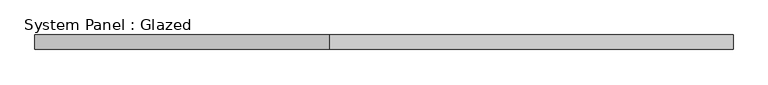
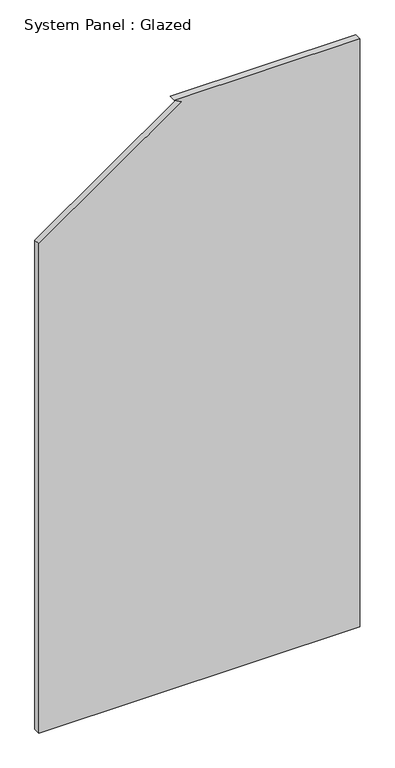
"""IFC4 building model written with IfcOpenShell, lengths in millimetres: plate geometry, System Panel : Glazed."""

from ifc_helpers import new_model, si_unit, frame, origin, place, context, project, spatial, polyline, outline, extrude, source, transform, mapped, element, save


def system_panel_glazed_7f2b43f2(model_context):
    return source(origin(), model_context, "Body", "SweptSolid", [
        extrude(outline(polyline([(0.0, -600.0), (0.0, 600.0), (2325.0, 600.0), (2325.0, -93.111196), (2309.0423978, -64.4323741), (1934.0339089, -600.0), (0.0, -600.0)])), frame((0.0, -49.5, 0.0), z_axis=(0.0, 1.0, 0.0), x_axis=(0.0, 0.0, 1.0)), (0.0, 0.0, 1.0), 25.0),
    ])


if __name__ == "__main__":
    model = new_model("IFC4")
    model_context = context("Model", 3, world=origin())
    ifc_project = project(units=[si_unit("LENGTHUNIT", "METRE", prefix="MILLI")], contexts=[model_context])
    site = spatial("IfcSite", under=ifc_project)
    building = spatial("IfcBuilding", under=site)
    placement = place(None, origin())
    system_panel_glazed_shape = system_panel_glazed_7f2b43f2(model_context)
    element("IfcPlate", 1, ObjectType="System Panel : Glazed", at=placement, inside=building, context=model_context, shape_type="MappedRepresentation", body=[
        mapped(system_panel_glazed_shape, transform((0.0, 0.0, 0.0), x_axis=(1.0, 0.0, 0.0), y_axis=(0.0, 1.0, 0.0), z_axis=(0.0, 0.0, 1.0))),
    ])
    save(model, "model.ifc")

# Revit data of these elements
# Type "System Panel : Glazed"
#   Construction Type Id = "GSP4R"
#   Analytic Construction = "1/8 in Pilkington single glazing"
#   Visual Light Transmittance = 0.9
#   Solar Heat Gain Coefficient = 0.86
#   Heat Transfer Coefficient (U) = 6.7069 W/(m²·K)
#   Define Thermal Properties by = 1
# Element 1 (IfcPlate, "System Panel : Glazed")
#   Materials on its faces: "Glass"
# Materials
#   "Glass": class "Glass", colour RGB 0 128 192, transparency 0.9, Description = "Soda Lime Glass", Cost = 0
